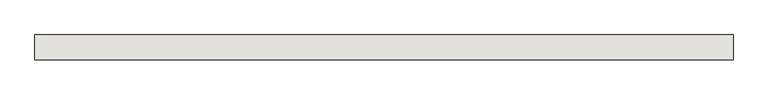
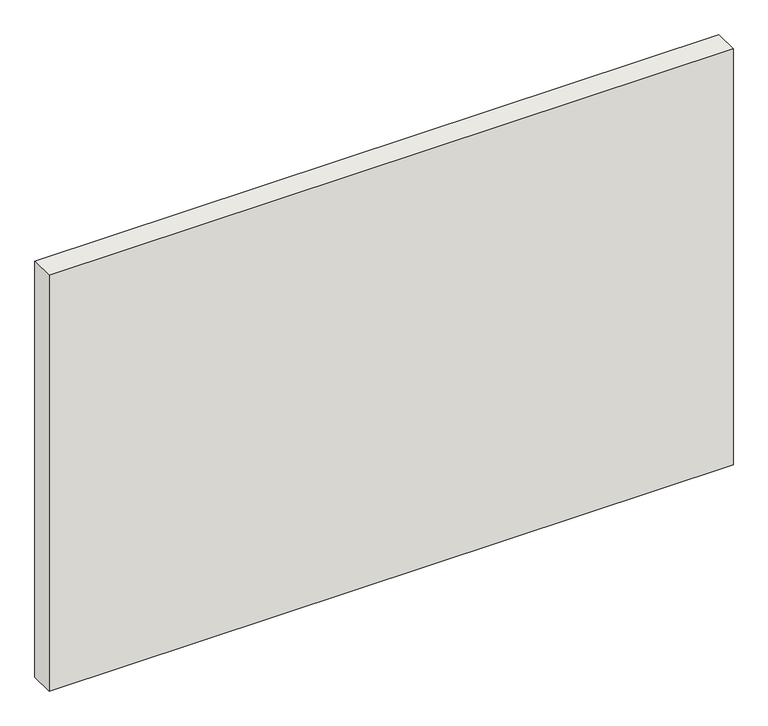
"""IFC4 building model written with IfcOpenShell, lengths in millimetres: wall geometry, Holzwand."""

from ifc_helpers import new_model, si_unit, origin, origin_with_axes, place, context, project, spatial, polyline, outline, extrude, source, transform, mapped, element, save


def wall_31205568(model_context):
    return source(origin(), model_context, "Body", "SweptSolid", [
        extrude(outline(polyline([(0.0, 50.0), (1401.2229627, 50.0), (1401.2229627, 0.0), (0.0, 0.0), (0.0, 50.0)])), origin_with_axes(), (0.0, 0.0, 1.0), 900.0),
    ])


if __name__ == "__main__":
    model = new_model("IFC4")
    model_context = context("Model", 3, world=origin())
    ifc_project = project(units=[si_unit("LENGTHUNIT", "METRE", prefix="MILLI")], contexts=[model_context])
    site = spatial("IfcSite", under=ifc_project)
    building = spatial("IfcBuilding", under=site)
    placement = place(None, origin())
    wall_shape = wall_31205568(model_context)
    element("IfcWall", 1, ObjectType="Holzwand", at=placement, inside=building, context=model_context, shape_type="MappedRepresentation", body=[
        mapped(wall_shape, transform((0.0, 0.0, 0.0), x_axis=(1.0, 0.0, 0.0), y_axis=(0.0, 1.0, 0.0), z_axis=(0.0, 0.0, 1.0))),
    ])
    save(model, "model.ifc")

# Revit data of these elements
# Element 1 (IfcWall, "Holzwand")
#   Materials on its faces: "holzschalung"
# Materials
#   "holzschalung": class "Unassigned", colour RGB 128 128 128, transparency 0
